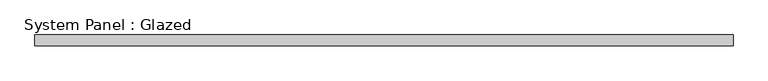
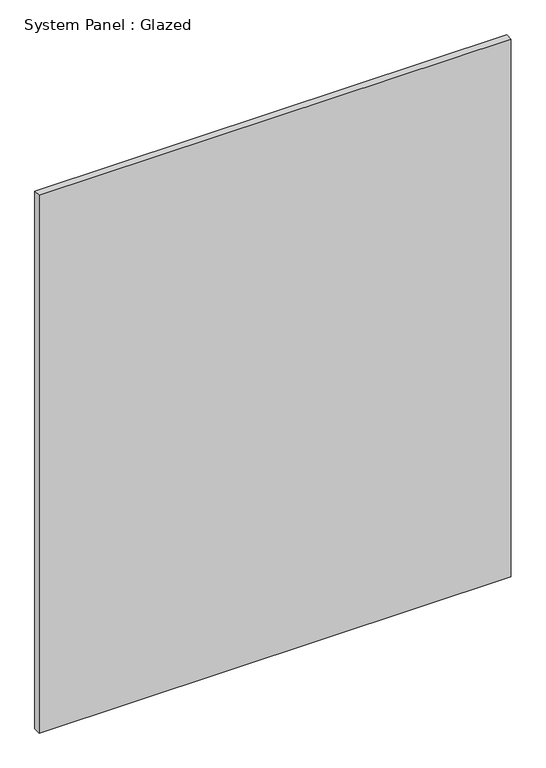
"""IFC4 building model written with IfcOpenShell, lengths in millimetres: plate geometry, System Panel : Glazed."""

from ifc_helpers import new_model, si_unit, origin, origin_with_axes, place, context, project, spatial, polyline, outline, extrude, source, transform, mapped, element, save


def system_panel_glazed_da9c9e0f(model_context):
    return source(origin(), model_context, "Body", "SweptSolid", [
        extrude(outline(polyline([(810.0, 24.5), (-810.0, 24.5), (-810.0, 49.5), (810.0, 49.5), (810.0, 24.5)])), origin_with_axes(), (0.0, 0.0, 1.0), 1950.0),
    ])


if __name__ == "__main__":
    model = new_model("IFC4")
    model_context = context("Model", 3, world=origin())
    ifc_project = project(units=[si_unit("LENGTHUNIT", "METRE", prefix="MILLI")], contexts=[model_context])
    site = spatial("IfcSite", under=ifc_project)
    building = spatial("IfcBuilding", under=site)
    placement = place(None, origin())
    system_panel_glazed_shape = system_panel_glazed_da9c9e0f(model_context)
    element("IfcPlate", 1, ObjectType="System Panel : Glazed", at=placement, inside=building, context=model_context, shape_type="MappedRepresentation", body=[
        mapped(system_panel_glazed_shape, transform((0.0, 0.0, 0.0), x_axis=(1.0, 0.0, 0.0), y_axis=(0.0, 1.0, 0.0), z_axis=(0.0, 0.0, 1.0))),
    ])
    save(model, "model.ifc")

# Revit data of these elements
# Element 1 (IfcPlate, "System Panel : Glazed")
#   Materials on its faces: "Glass"
# Materials
#   "Glass": class "Glass", colour RGB 0 128 192, transparency 0.9
